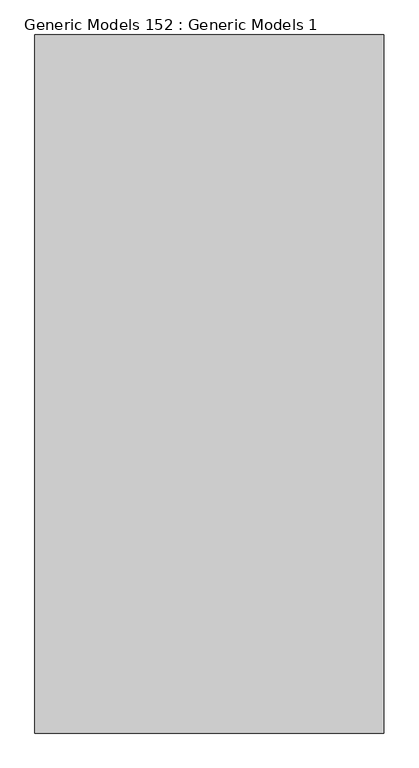
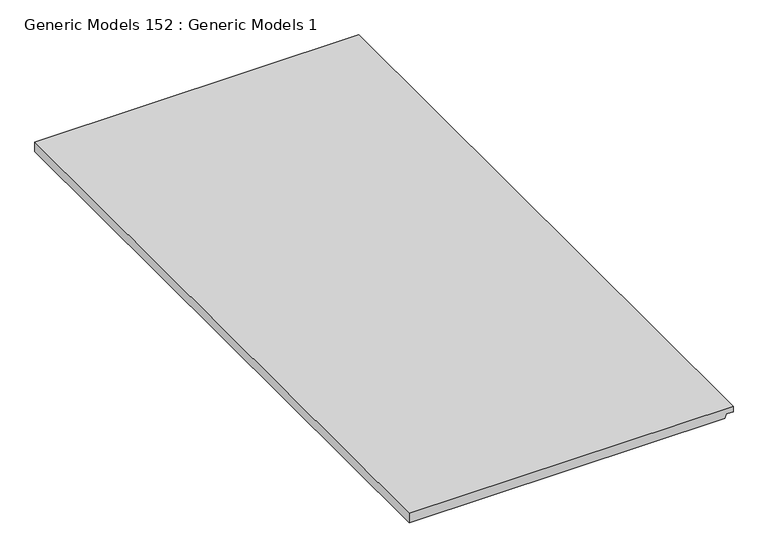
"""IFC4 building model written with IfcOpenShell, lengths in millimetres: proxy geometry, Generic Models 152 : Generic Models 1."""

from ifc_helpers import new_model, si_unit, frame, origin, place, context, project, spatial, polyline, outline, extrude, source, transform, mapped, element, save


def generic_models_152_generic_models_1_24b688b4(model_context):
    return source(origin(), model_context, "Body", "SweptSolid", [
        extrude(outline(polyline([(2253.330428, 51977.6676133), (2253.330428, 51368.0676133), (2234.280428, 51368.0676133), (2234.280428, 51962.0785996), (2242.217928, 51964.9676133), (2242.217928, 51977.6676133), (2253.330428, 51977.6676133)])), frame((0.0, 0.0, 0.0), z_axis=(0.0, 1.0, 0.0), x_axis=(0.0, 0.0, 1.0)), (0.0, 0.0, 1.0), 1219.2),
    ])


if __name__ == "__main__":
    model = new_model("IFC4")
    model_context = context("Model", 3, world=origin())
    ifc_project = project(units=[si_unit("LENGTHUNIT", "METRE", prefix="MILLI")], contexts=[model_context])
    site = spatial("IfcSite", under=ifc_project)
    building = spatial("IfcBuilding", under=site)
    placement = place(None, origin())
    generic_models_152_generic_models_1_shape = generic_models_152_generic_models_1_24b688b4(model_context)
    element("IfcBuildingElementProxy", 1, Name="Generic Models 152 : Generic Models 1", ObjectType="Generic Models 152 : Generic Models 1", at=placement, inside=building, context=model_context, shape_type="MappedRepresentation", body=[
        mapped(generic_models_152_generic_models_1_shape, transform((0.0, 0.0, 0.0), x_axis=(1.0, 0.0, 0.0), y_axis=(0.0, 1.0, 0.0), z_axis=(0.0, 0.0, 1.0))),
    ])
    save(model, "model.ifc")

# Revit data of these elements
# Element 1 (IfcBuildingElementProxy, "Generic Models 152 : Generic Models 1")
#   Materials on its faces: "CEILING AS SCHEDULED"
# Materials
#   "CEILING AS SCHEDULED": class "Generic", colour RGB 255 255 255, transparency 0, Cost = 0
